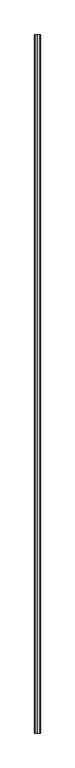
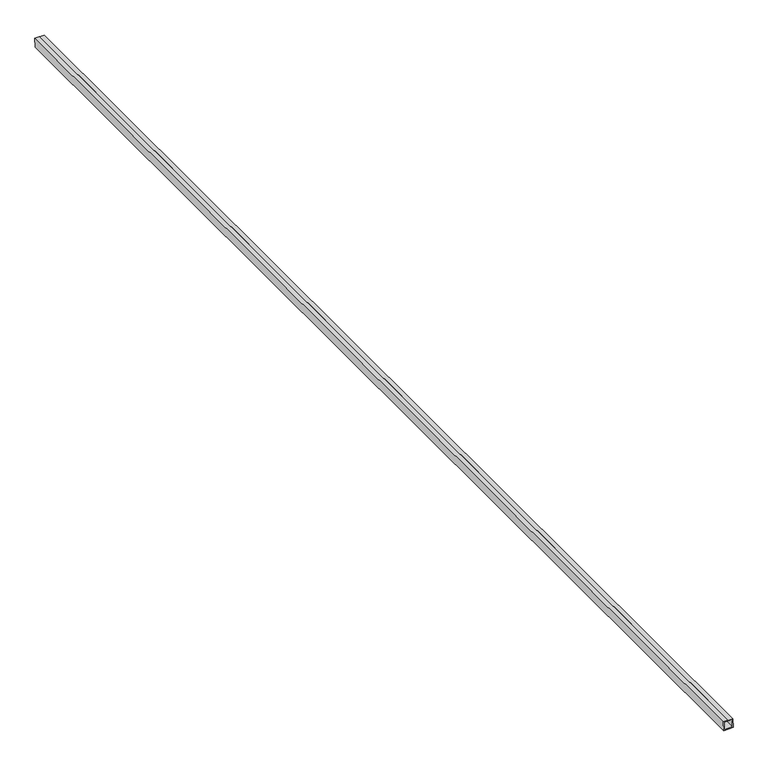
"""IFC4 building model written with IfcOpenShell, lengths in millimetres: proxy geometry, Inner panel:Inner panel:1:Inner panel:1 : Inner panel:Inner panel:300324:2:Inner panel:1:Inner panel:1 : Inner panel:Inner panel:300324:2 : Inner panel:Inner panel:1:Inner panel:1 : Inner panel:Inner panel:300324:300043:34 : Inner panel:Inner panel:1:Inner panel:1 : Inner panel:Inner panel:300324:2:Inner panel:1:Inner panel:1 : Inner panel:Inner panel:300324:2 : Inner panel:Inner panel:1:Inner panel:1 : Inner panel:Inner panel:300324:300043:308120."""

from ifc_helpers import new_model, si_unit, frame, origin, place, context, project, spatial, polyline, outline, extrude, source, transform, mapped, element, save


def generic_models_20bc129d(model_context):
    return source(origin(), model_context, "Body", "SweptSolid", [
        extrude(outline(polyline([(3888.1950703, 558884.7829759), (3885.8158846, 558884.8821086), (3886.4767695, 558900.7433462), (3853.1681707, 558902.1312045), (3851.7803124, 558868.8226056), (3885.0889112, 558867.4347474), (3885.7497961, 558883.2959849), (3888.1289818, 558883.1968522), (3887.3689641, 558864.956429), (3849.3019941, 558866.5425527), (3850.8881178, 558904.6095228), (3888.9550879, 558903.0233991), (3888.1950703, 558884.7829759)])), frame((0.0, -575657.416384, 0.0), z_axis=(0.0, 1.0, 0.0), x_axis=(0.0, 0.0, 1.0)), (0.0, 0.0, 1.0), 4876.8),
    ])


if __name__ == "__main__":
    model = new_model("IFC4")
    model_context = context("Model", 3, world=origin())
    ifc_project = project(units=[si_unit("LENGTHUNIT", "METRE", prefix="MILLI")], contexts=[model_context])
    site = spatial("IfcSite", under=ifc_project)
    building = spatial("IfcBuilding", under=site)
    placement = place(None, origin())
    generic_models_shape = generic_models_20bc129d(model_context)
    element("IfcBuildingElementProxy", 1, Name="Inner panel:Inner panel:1:Inner panel:1 : Inner panel:Inner panel:300324:2:Inner panel:1:Inner panel:1 : Inner panel:Inner panel:300324:2 : Inner panel:Inner panel:1:Inner panel:1 : Inner panel:Inner panel:300324:300043:34 : Inner panel:Inner panel:1:Inner panel:1 : Inner panel:Inner panel:300324:2:Inner panel:1:Inner panel:1 : Inner panel:Inner panel:300324:2 : Inner panel:Inner panel:1:Inner panel:1 : Inner panel:Inner panel:300324:300043:308120", ObjectType="Inner panel:Inner panel:1:Inner panel:1 : Inner panel:Inner panel:300324:2:Inner panel:1:Inner panel:1 : Inner panel:Inner panel:300324:2 : Inner panel:Inner panel:1:Inner panel:1 : Inner panel:Inner panel:300324:300043:34 : Inner panel:Inner panel:1:Inner panel:1 : Inner panel:Inner panel:300324:2:Inner panel:1:Inner panel:1 : Inner panel:Inner panel:300324:2 : Inner panel:Inner panel:1:Inner panel:1 : Inner panel:Inner panel:300324:300043:308120", at=placement, inside=building, context=model_context, shape_type="MappedRepresentation", body=[
        mapped(generic_models_shape, transform((0.0, 0.0, 0.0), x_axis=(1.0, 0.0, 0.0), y_axis=(0.0, 1.0, 0.0), z_axis=(0.0, 0.0, 1.0))),
    ])
    save(model, "model.ifc")

# Revit data of these elements
# Type "Inner panel:Inner panel:1:Inner panel:1 : Inner panel:Inner panel:300324:2:Inner panel:1:Inner panel:1 : Inner panel:Inner panel:300324:2 : Inner panel:Inner panel:1:Inner panel:1 : Inner panel:Inner panel:300324:300043:34 : Inner panel:Inner panel:1:Inner panel:1 : Inner panel:Inner panel:300324:2:Inner panel:1:Inner panel:1 : Inner panel:Inner panel:300324:2 : Inner panel:Inner panel:1:Inner panel:1 : Inner panel:Inner panel:300324:300043:308120"
#   NameOverride = "Inner panel:Inner panel:1:Inner panel:1 : Inner panel:Inner panel:300324:2:Inner panel:1:Inner panel:1 : Inner panel:Inner panel:300324:2 : Inner panel:Inner panel:1:Inner panel:1 : Inner panel:Inner panel:300324:300043:308120"
#   ObjectTypeOverride = "Inner panel:1:Inner panel:1 : Inner panel:Inner panel:300324:2 : Inner panel:Inner panel:1:Inner panel:1 : Inner panel:Inner panel:300324:300043"
#   Reference = "Inner panel"
#   Tag = "308120"
# Element 1 (IfcBuildingElementProxy, "Inner panel:Inner panel:1:Inner panel:1 : Inner panel:Inner panel:300324:2:Inner panel:1:Inner panel:1 : Inner panel:Inner panel:300324:2 : Inner panel:Inner panel:1:Inner panel:1 : Inner panel:Inner panel:300324:300043:34 : Inner panel:Inner panel:1:Inner panel:1 : Inner panel:Inner panel:300324:2:Inner panel:1:Inner panel:1 : Inner panel:Inner panel:300324:2 : Inner panel:Inner panel:1:Inner panel:1 : Inner panel:Inner panel:300324:300043:308120")
#   Materials on its faces: "1 1/2\" X 1 1/2\" x 1/8\" ALUM. TUBE (6061-T6) - (2) #16 WOOD SCREWS WITH 2.5\" EMBED AT EACH GLULAM - (1) SCREW AT ENDS"
# Materials
#   "1 1/2\" X 1 1/2\" x 1/8\" ALUM. TUBE (6061-T6) - (2) #16 WOOD SCREWS WITH 2.5\" EMBED AT EACH GLULAM - (1) SCREW AT ENDS": class "Unassigned", colour RGB 202 201 200, transparency 0, Cost = 0
